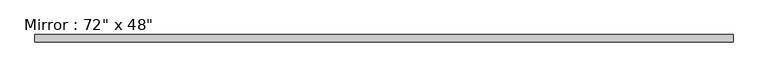
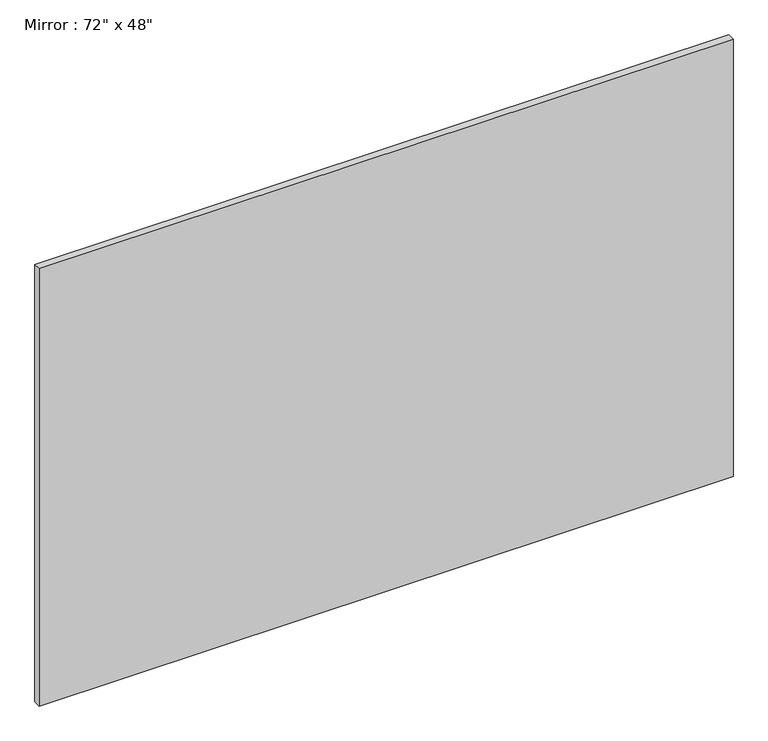
"""IFC4 building model written with IfcOpenShell, lengths in millimetres: proxy geometry."""

import ifcopenshell
import ifcopenshell.guid

model = None  # the IFC model being written
_history = None  # IfcOwnerHistory: only IFC2X3 demands one
_inside = {}  # id of a spatial element -> (the spatial element, [elements in it])
_under = {}  # id of a project, library or spatial element -> (it, [spatial elements below it])
_declared = {}  # id of a project -> (the project, [libraries it declares])
_typed = {}  # id of a type object -> (the type object, [elements of that type])
_made_of = {}  # id of a material, layer set ... -> (it, [elements and type objects made of it])


def new_model(schema):
    """Start an empty IFC model of exactly this schema.

    Asked for "IFC4X3", IfcOpenShell would pick the latest addendum, in which some entities
    have other attributes; the version numbers below select the first issue.
    IFC2X3 requires an IfcOwnerHistory on every rooted entity: one is made here for all.
    """
    global model, _history
    if schema == "IFC4X3":
        model = ifcopenshell.file(schema_version=(4, 3, 0, 0))
    else:
        model = ifcopenshell.file(schema=schema)
    _inside.clear()
    _under.clear()
    _declared.clear()
    _typed.clear()
    _made_of.clear()
    _history = None
    if model.schema == "IFC2X3":
        org = make("IfcOrganization", Name="unknown")
        user = make(
            "IfcPersonAndOrganization",
            ThePerson=make("IfcPerson", FamilyName="unknown"),
            TheOrganization=org,
        )
        app = make(
            "IfcApplication",
            ApplicationDeveloper=org,
            Version="unknown",
            ApplicationFullName="unknown",
            ApplicationIdentifier="unknown",
        )
        _history = make(
            "IfcOwnerHistory",
            OwningUser=user,
            OwningApplication=app,
            ChangeAction="ADDED",
            CreationDate=0,
        )
    return model


def make(cls, **values):
    """One entity of the class cls with the attributes given. An attribute that is None is left unset."""
    return model.create_entity(
        cls, **{name: value for name, value in values.items() if value is not None}
    )


def rooted(cls, **values):
    """An entity with a GlobalId (a new one), such as an element, a storey or a relation."""
    return make(cls, GlobalId=ifcopenshell.guid.new(), OwnerHistory=_history, **values)


def si_unit(unit_type, name, prefix=None):
    """IfcSIUnit, for example si_unit("LENGTHUNIT", "METRE", prefix="MILLI")."""
    return make("IfcSIUnit", UnitType=unit_type, Prefix=prefix, Name=name)


def assignment(units):
    """IfcUnitAssignment: the units of a project."""
    return None if units is None else make("IfcUnitAssignment", Units=units)


def point(xyz):
    """IfcCartesianPoint."""
    return None if xyz is None else make("IfcCartesianPoint", Coordinates=xyz)


def direction(xyz):
    """IfcDirection."""
    return None if xyz is None else make("IfcDirection", DirectionRatios=xyz)


def frame(location, z_axis=None, x_axis=None):
    """IfcAxis2Placement3D, a coordinate frame: its origin and axes. An axis left out is left unset."""
    return make(
        "IfcAxis2Placement3D",
        Location=point(location),
        Axis=direction(z_axis),
        RefDirection=direction(x_axis),
    )


def origin():
    """The frame at (0, 0, 0) with its axes left unset."""
    return frame((0.0, 0.0, 0.0))


def place(relative_to, where):
    """IfcLocalPlacement: puts the frame where relative to a parent placement (None: the world)."""
    return make(
        "IfcLocalPlacement", PlacementRelTo=relative_to, RelativePlacement=where
    )


def context(
    kind, dimensions, precision=None, world=None, true_north=None, identifier=None
):
    """IfcGeometricRepresentationContext, for example the 3D "Model" context."""
    return make(
        "IfcGeometricRepresentationContext",
        ContextIdentifier=identifier,
        ContextType=kind,
        CoordinateSpaceDimension=dimensions,
        Precision=precision,
        WorldCoordinateSystem=world,
        TrueNorth=true_north,
    )


def project(units=None, contexts=None):
    """IfcProject with its units and contexts."""
    return rooted(
        "IfcProject",
        Name="project",
        RepresentationContexts=contexts,
        UnitsInContext=assignment(units),
    )


def spatial(cls, under=None, at=None, **own):
    """A site, building, storey or space (cls), placed at a placement, below another one or the project."""
    s = rooted(cls, ObjectPlacement=at, **own)
    if under is not None:
        _under.setdefault(under.id(), (under, []))[1].append(s)
    return s


def polyline(points):
    """IfcPolyline through the points."""
    return make("IfcPolyline", Points=[point(p) for p in points])


def outline(outer, holes=None, kind="AREA"):
    """IfcArbitraryClosedProfileDef: a profile drawn as a closed curve; with holes, ...WithVoids."""
    if holes is None:
        return make("IfcArbitraryClosedProfileDef", ProfileType=kind, OuterCurve=outer)
    return make(
        "IfcArbitraryProfileDefWithVoids",
        ProfileType=kind,
        OuterCurve=outer,
        InnerCurves=holes,
    )


def extrude(swept, where, along, depth):
    """IfcExtrudedAreaSolid: the profile swept, set in the frame where, extruded along a direction by depth."""
    return make(
        "IfcExtrudedAreaSolid",
        SweptArea=swept,
        Position=where,
        ExtrudedDirection=direction(along),
        Depth=depth,
    )


def shape(context_of_items, identifier, shape_type, items):
    """IfcShapeRepresentation: the items that make up one representation, for example the "Body"."""
    return make(
        "IfcShapeRepresentation",
        ContextOfItems=context_of_items,
        RepresentationIdentifier=identifier,
        RepresentationType=shape_type,
        Items=items,
    )


def source(mapping_origin, context_of_items, identifier, shape_type, items):
    """IfcRepresentationMap: a shape defined once, which mapped items show again and again."""
    return make(
        "IfcRepresentationMap",
        MappingOrigin=mapping_origin,
        MappedRepresentation=shape(context_of_items, identifier, shape_type, items),
    )


def transform(
    local_origin,
    x_axis=None,
    y_axis=None,
    z_axis=None,
    scale=None,
    scale2=None,
    scale3=None,
    uniform=True,
):
    """IfcCartesianTransformationOperator3D, or its non-uniform kind. x_axis, y_axis, z_axis: its Axis1, 2, 3."""
    if uniform:
        return make(
            "IfcCartesianTransformationOperator3D",
            Axis1=direction(x_axis),
            Axis2=direction(y_axis),
            LocalOrigin=point(local_origin),
            Scale=scale,
            Axis3=direction(z_axis),
        )
    return make(
        "IfcCartesianTransformationOperator3DnonUniform",
        Axis1=direction(x_axis),
        Axis2=direction(y_axis),
        LocalOrigin=point(local_origin),
        Scale=scale,
        Axis3=direction(z_axis),
        Scale2=scale2,
        Scale3=scale3,
    )


def mapped(mapping_source, mapping_target):
    """IfcMappedItem: shows the shape of a source again, moved by a transform."""
    return make(
        "IfcMappedItem", MappingSource=mapping_source, MappingTarget=mapping_target
    )


def made_of(thing, what):
    """Note that an element or type object is made of a material, layer set ...; save() writes the relation."""
    if what is not None:
        _made_of.setdefault(what.id(), (what, []))[1].append(thing)
    return thing


def element(
    cls,
    number,
    at=None,
    inside=None,
    cuts=None,
    type_object=None,
    material=None,
    context=None,
    identifier="Body",
    shape_type=None,
    held_by="IfcProductDefinitionShape",
    body=None,
    shapes=None,
    **own,
):
    """One element of the class cls, such as IfcWall. Its Tag is "e" and its number.

    at: its placement. inside: the storey or other place that contains it. cuts: it is an
    opening in that element (IfcRelVoidsElement). A single representation is given by context,
    identifier, shape_type and body (its items); several are given by shapes. held_by: the class
    of the entity that holds the representations. save() writes the other relations.
    """
    e = rooted(cls, Tag="e%d" % number, ObjectPlacement=at, **own)
    if body is not None:
        shapes = [shape(context, identifier, shape_type, body)]
    if shapes is not None:
        e.Representation = make(held_by, Representations=shapes)
    if inside is not None:
        _inside.setdefault(inside.id(), (inside, []))[1].append(e)
    if cuts is not None:
        rooted(
            "IfcRelVoidsElement", RelatingBuildingElement=cuts, RelatedOpeningElement=e
        )
    if type_object is not None:
        _typed.setdefault(type_object.id(), (type_object, []))[1].append(e)
    return made_of(e, material)


def aggregate(whole, parts):
    """IfcRelAggregates: a whole, such as a stair, and the parts it consists of."""
    return rooted("IfcRelAggregates", RelatingObject=whole, RelatedObjects=parts)


def save(model, path):
    """Write the relations noted so far, then the file.

    IfcRelAggregates (storeys below a building ...), IfcRelContainedInSpatialStructure (elements
    in a storey), IfcRelDefinesByType, IfcRelAssociatesMaterial and IfcRelDeclares: one each for
    every whole, place, type object, material and project.
    """
    for whole, parts in _under.values():
        aggregate(whole, parts)
    for where, things in _inside.values():
        rooted(
            "IfcRelContainedInSpatialStructure",
            RelatedElements=things,
            RelatingStructure=where,
        )
    for kind, things in _typed.values():
        rooted("IfcRelDefinesByType", RelatedObjects=things, RelatingType=kind)
    for what, things in _made_of.values():
        rooted("IfcRelAssociatesMaterial", RelatedObjects=things, RelatingMaterial=what)
    for by, libraries in _declared.values():
        rooted("IfcRelDeclares", RelatingContext=by, RelatedDefinitions=libraries)
    model.write(path)


def proxy_95b4f9e6(model_context):
    return source(origin(), model_context, "Body", "SweptSolid", [
        extrude(outline(polyline([(-889.9296989, 82.55), (938.8703011, 82.55), (938.8703011, 63.5), (-889.9296989, 63.5), (-889.9296989, 82.55)])), frame((0.0, 0.0, 1066.8), z_axis=(0.0, 0.0, 1.0), x_axis=(1.0, 0.0, 0.0)), (0.0, 0.0, 1.0), 1219.2),
    ])


if __name__ == "__main__":
    model = new_model("IFC4")
    model_context = context("Model", 3, world=origin())
    ifc_project = project(units=[si_unit("LENGTHUNIT", "METRE", prefix="MILLI")], contexts=[model_context])
    site = spatial("IfcSite", under=ifc_project)
    building = spatial("IfcBuilding", under=site)
    placement = place(None, origin())
    proxy_shape = proxy_95b4f9e6(model_context)
    element("IfcBuildingElementProxy", 1, Name="Mirror : 72\" x 48\"", ObjectType="Mirror : 72\" x 48\"", at=placement, inside=building, context=model_context, shape_type="MappedRepresentation", body=[
        mapped(proxy_shape, transform((0.0, 0.0, 0.0), x_axis=(1.0, 0.0, 0.0), y_axis=(0.0, 1.0, 0.0), z_axis=(0.0, 0.0, 1.0))),
    ])
    save(model, "model.ifc")

# Revit data of these elements
# Type "Mirror : 72\" x 48\""
#   Assembly Code = "C1030200"
#   Height = 4' - 0"
#   Mounting Height = 3' - 6"
#   Width = 6' - 0"
#   Default Elevation = 0
# Element 1 (IfcBuildingElementProxy, "Mirror : 72\" x 48\"")
#   Materials on its faces: "Mirror"
# Materials
#   "Mirror": class "Glass", colour RGB 120 120 120, transparency 0, Description = "Mirror glass", Cost = 0
